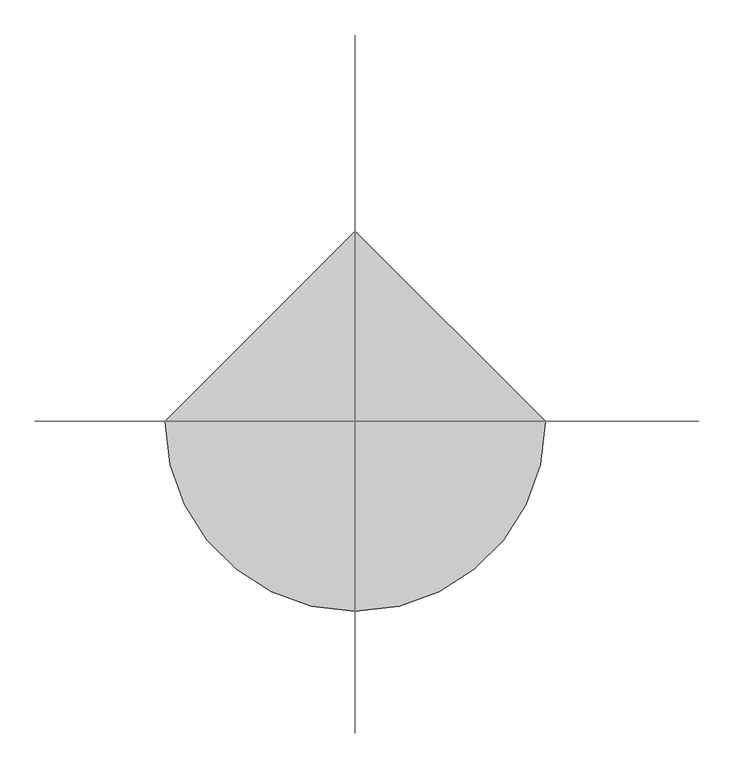
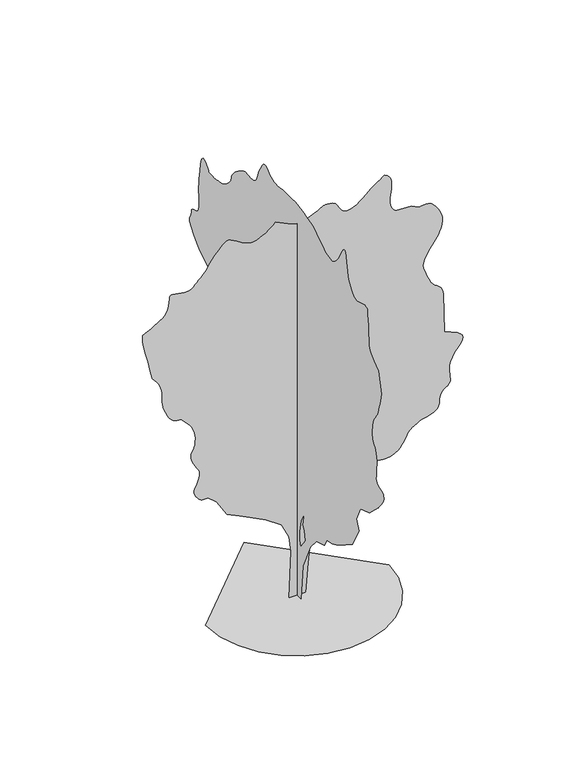
"""IFC4 building model written with IfcOpenShell, lengths in millimetres: proxy geometry, honeylocust 26170 : honeylocust 26170."""

from ifc_helpers import new_model, si_unit, origin, place, context, project, spatial, triangles, source, transform, mapped, element, save


def entourage_cc46a1f1(model_context):
    return source(origin(), model_context, "Body", "Tessellation", [
        triangles([(0.0017564, 138.2462219, 0.0), (0.0017564, -127.0105432, 0.0), (0.0017564, -184.6753374, 668.9082985), (0.0017564, -426.8668951, 1176.3566122), (0.0017564, -611.3926231, 1395.4822632), (0.0017564, -865.1155083, 1476.2135273), (0.0017564, -934.3152088, 1614.6078415), (0.0017564, -1118.8409369, 1660.7391827), (0.0017564, -1168.1321142, 1679.0297813), (0.0017564, -1234.9772346, 1712.4509972), (0.0017564, -1316.4476978, 1758.4833618), (0.0017564, -1409.6173016, 1814.6021748), (0.0017564, -1511.5651485, 1878.2849155), (0.0017564, -1619.3626385, 1947.0122612), (0.0017564, -1730.0862579, 2018.2590752), (0.0017564, -1937.6776566, 2398.8447109), (0.0017564, -1856.9463924, 2583.3806854), (0.0017564, -1983.8091431, 2848.632518), (0.0017564, -2272.1318058, 2952.4168808), (0.0017564, -2537.389016, 3206.1371498), (0.0017564, -2543.9089668, 3214.0110878), (0.0017564, -2561.3334846, 3235.1946785), (0.0017564, -2586.4031754, 3266.0558762), (0.0017564, -2615.9435234, 3302.9873428), (0.0017564, -2646.6774033, 3342.3317436), (0.0017564, -2675.3794304, 3380.4573235), (0.0017564, -2698.8489281, 3413.7311646), (0.0017564, -2714.4444878, 3444.5414932), (0.0017564, -2721.9882133, 3476.5453537), (0.0017564, -2721.8358971, 3508.1684235), (0.0017564, -2714.4444878, 3537.73377), (0.0017564, -2700.1950668, 3563.6926506), (0.0017564, -2679.4940048, 3584.4190018), (0.0017564, -2652.7226738, 3598.2620522), (0.0017564, -2621.3536583, 3608.345739), (0.0017564, -2588.1556847, 3619.6488281), (0.0017564, -2555.5675575, 3633.3648514), (0.0017564, -2526.024884, 3650.7129204), (0.0017564, -2501.9153091, 3672.9124374), (0.0017564, -2485.67444, 3701.157225), (0.0017564, -2479.7233498, 3736.6663948), (0.0017564, -2481.5749809, 3780.2273987), (0.0017564, -2486.0453476, 3831.0780739), (0.0017564, -2491.5266991, 3887.9740196), (0.0017564, -2496.4008202, 3949.6961243), (0.0017564, -2499.0579254, 4015.0755638), (0.0017564, -2497.8818344, 4082.8426483), (0.0017564, -2491.2575294, 4151.8544243), (0.0017564, -2477.5720276, 4213.7541344), (0.0017564, -2458.0368828, 4262.9284584), (0.0017564, -2435.2733013, 4302.24757), (0.0017564, -2411.9053963, 4334.4801956), (0.0017564, -2390.5542286, 4362.4965088), (0.0017564, -2373.8434753, 4389.0902344), (0.0017564, -2364.3947788, 4417.1062569), (0.0017564, -2359.5864967, 4450.1263344), (0.0017564, -2355.5860142, 4489.1913918), (0.0017564, -2353.1983692, 4533.3113731), (0.0017564, -2353.2315067, 4581.4694801), (0.0017564, -2356.4927902, 4632.6250786), (0.0017564, -2363.7901646, 4685.8128204), (0.0017564, -2375.9288132, 4740.016198), (0.0017564, -2392.0679443, 4787.9461212), (0.0017564, -2410.4271435, 4825.3601166), (0.0017564, -2430.3991802, 4855.916391), (0.0017564, -2451.3794403, 4883.2722794), (0.0017564, -2472.7636002, 4911.0089584), (0.0017564, -2493.9471909, 4942.7843445), (0.0017564, -2514.3232727, 4982.2051941), (0.0017564, -2534.0944496, 5031.4045166), (0.0017564, -2553.8659172, 5089.0626251), (0.0017564, -2573.6269203, 5153.8075104), (0.0017564, -2593.4135033, 5224.1654251), (0.0017564, -2613.1747971, 5298.7905212), (0.0017564, -2632.9360909, 5376.2096329), (0.0017564, -2652.7226738, 5455.0763306), (0.0017564, -2548.9127312, 5835.6443802), (0.0017564, -2410.52612, 5939.4537415), (0.0017564, -2376.165136, 5966.8602081), (0.0017564, -2343.2136589, 5995.5625259), (0.0017564, -2313.0867188, 6026.9059616), (0.0017564, -2287.1965839, 6062.1863663), (0.0017564, -2266.9553776, 6102.6995911), (0.0017564, -2253.772752, 6149.7659042), (0.0017564, -2249.0662079, 6204.705574), (0.0017564, -2247.7225399, 6269.3992996), (0.0017564, -2243.9556187, 6343.7709229), (0.0017564, -2238.1721054, 6426.2187973), (0.0017564, -2230.7756092, 6515.1186035), (0.0017564, -2222.1675591, 6608.8704391), (0.0017564, -2212.7518547, 6705.8220795), (0.0017564, -2202.9347214, 6804.4247818), (0.0017564, -2185.5179066, 6814.1270966), (0.0017564, -2167.3950302, 6822.8393555), (0.0017564, -2147.8598854, 6829.5453415), (0.0017564, -2126.2064106, 6833.2026764), (0.0017564, -2101.7285442, 6832.8218857), (0.0017564, -2073.7199341, 6827.4117508), (0.0017564, -2041.4746639, 6815.9560547), (0.0017564, -2006.8748863, 6801.3255524), (0.0017564, -1972.2775795, 6787.914743), (0.0017564, -1937.6776566, 6776.9165771), (0.0017564, -1903.077879, 6769.5501663), (0.0017564, -1868.4805721, 6767.0357849), (0.0017564, -1833.8806492, 6770.5663834), (0.0017564, -1799.2833424, 6781.3616547), (0.0017564, -1765.6919334, 6801.5546082), (0.0017564, -1733.9191635, 6831.4504578), (0.0017564, -1703.6576385, 6869.42314), (0.0017564, -1674.6050514, 6913.8221741), (0.0017564, -1646.4618565, 6963.0982361), (0.0017564, -1618.9257465, 7015.5746841), (0.0017564, -1591.689473, 7069.6766144), (0.0017564, -1522.4922432, 7484.8646439), (0.0017564, -1510.0182953, 7494.262326), (0.0017564, -1496.8382858, 7500.8665741), (0.0017564, -1482.2460079, 7501.8060516), (0.0017564, -1465.5354, 7494.262326), (0.0017564, -1446.0002552, 7475.4413818), (0.0017564, -1422.9345119, 7442.4974625), (0.0017564, -1395.6321087, 7392.5865555), (0.0017564, -1366.480545, 7335.9952423), (0.0017564, -1337.5296959, 7284.4588531), (0.0017564, -1307.5703327, 7237.3669601), (0.0017564, -1275.393663, 7194.085881), (0.0017564, -1239.7855167, 7154.0296051), (0.0017564, -1199.5366653, 7116.6156097), (0.0017564, -1153.4407871, 7081.2078873), (0.0017564, -1100.9873028, 7057.7133911), (0.0017564, -1043.0880753, 7054.1827927), (0.0017564, -980.6472645, 7067.2889694), (0.0017564, -914.5768787, 7093.7047989), (0.0017564, -845.7836214, 7130.1287384), (0.0017564, -775.1741959, 7173.2069229), (0.0017564, -703.6555235, 7219.6128113), (0.0017564, -659.2741482, 7251.5405136), (0.0017564, -615.4946983, 7282.3758408), (0.0017564, -572.9269114, 7311.0014191), (0.0017564, -532.1751838, 7336.2748764), (0.0017564, -493.8440932, 7357.1282547), (0.0017564, -458.5406522, 7372.4186005), (0.0017564, -426.8668951, 7381.0547012), (0.0017564, -379.7931333, 7391.6464966), (0.0017564, -304.4771091, 7410.7220764), (0.0017564, -210.8004869, 7434.013678), (0.0017564, -108.6519436, 7457.3308594), (0.0017564, -7.915369, 7476.3808594), (0.0017564, 81.5235032, 7486.9726547), (0.0017564, 149.779584, 7484.8646439), (0.0017564, 204.0816928, 7478.1336594), (0.0017564, 257.9799291, 7476.2541229), (0.0017564, 311.0709472, 7476.9907059), (0.0017564, 362.9529548, 7478.1336594), (0.0017564, 413.2194723, 7477.4732346), (0.0017564, 461.4692888, 7472.7485229), (0.0017564, 507.2984682, 7461.8015167), (0.0017564, 555.4821914, 7451.6666702), (0.0017564, 608.9110522, 7450.0156082), (0.0017564, 664.3541433, 7455.4513229), (0.0017564, 718.5906584, 7466.5000671), (0.0017564, 768.3873281, 7481.7909943), (0.0017564, 810.5182594, 7499.9265152), (0.0017564, 841.7526175, 7519.4590439), (0.0017564, 869.6950979, 7543.2081757), (0.0017564, 902.8827524, 7570.9704346), (0.0017564, 939.4967966, 7596.9293152), (0.0017564, 977.728838, 7615.2171524), (0.0017564, 1015.7551506, 7619.9924423), (0.0017564, 1051.7671967, 7605.3875198), (0.0017564, 1083.943939, 7565.5858795), (0.0017564, 1111.584185, 7516.9952408), (0.0017564, 1135.5896965, 7477.701709), (0.0017564, 1156.5725727, 7444.2496811), (0.0017564, 1175.132341, 7413.2114594), (0.0017564, 1191.8760138, 7381.1564392), (0.0017564, 1207.410676, 7344.6819214), (0.0017564, 1222.3407967, 7300.3334656), (0.0017564, 1236.6967518, 7254.9693741), (0.0017564, 1251.0554684, 7217.07285), (0.0017564, 1266.8236919, 7185.6526749), (0.0017564, 1285.4164524, 7159.6432159), (0.0017564, 1308.248489, 7138.103833), (0.0017564, 1336.7269833, 7119.9683121), (0.0017564, 1372.2666744, 7104.2710144), (0.0017564, 1413.6914715, 7095.1529663), (0.0017564, 1457.9408054, 7094.9239105), (0.0017564, 1503.6022625, 7099.7247803), (0.0017564, 1549.2612488, 7105.7447617), (0.0017564, 1593.5105827, 7109.1480423), (0.0017564, 1634.9353798, 7106.0999725), (0.0017564, 1672.1235168, 7092.7397415), (0.0017564, 1714.3205051, 7068.3051865), (0.0017564, 1768.2192501, 7035.5897415), (0.0017564, 1828.5747231, 6996.1944717), (0.0017564, 1890.1391338, 6951.7954376), (0.0017564, 1947.6700699, 6903.9419632), (0.0017564, 1995.9198864, 6854.2845291), (0.0017564, 2029.6434093, 6804.4247818), (0.0017564, 2047.5985634, 6762.5657089), (0.0017564, 2056.0720287, 6732.1873306), (0.0017564, 2061.1140175, 6707.879512), (0.0017564, 2068.7821541, 6684.1809586), (0.0017564, 2085.1219997, 6655.6315384), (0.0017564, 2116.1913242, 6616.7949554), (0.0017564, 2168.0377235, 6562.2360764), (0.0017564, 2230.1762272, 6507.9306702), (0.0017564, 2288.0754547, 6470.9736237), (0.0017564, 2341.7380222, 6447.5297058), (0.0017564, 2391.1637844, 6433.7881027), (0.0017564, 2436.3553574, 6425.8885849), (0.0017564, 2477.3077995, 6419.9959213), (0.0017564, 2514.0259071, 6412.2998795), (0.0017564, 2553.510125, 6405.0352066), (0.0017564, 2599.6366699, 6402.2161926), (0.0017564, 2647.7694878, 6402.6225632), (0.0017564, 2693.3117661, 6405.0352066), (0.0017564, 2731.5640823, 6408.2611725), (0.0017564, 2757.9293335, 6411.0807678), (0.0017564, 2767.7589661, 6412.2998795), (0.0017564, 2779.3922676, 6430.4609802), (0.0017564, 2809.9738312, 6472.8281616), (0.0017564, 2853.0775955, 6521.2403229), (0.0017564, 2902.2519196, 6557.5625244), (0.0017564, 2950.9945839, 6563.6075043), (0.0017564, 2992.9045258, 6521.2403229), (0.0017564, 3021.4792351, 6412.2998795), (0.0017564, 3039.1830963, 6281.2613663), (0.0017564, 3053.0770157, 6180.2965988), (0.0017564, 3063.5417839, 6102.7251709), (0.0017564, 3070.9584824, 6041.8916748), (0.0017564, 3075.7846413, 5991.1680267), (0.0017564, 3078.3751808, 5943.8482407), (0.0017564, 3079.1373436, 5893.3274872), (0.0017564, 3077.918232, 5838.9459229), (0.0017564, 3075.0986366, 5784.5899384), (0.0017564, 3071.8729614, 5730.2089554), (0.0017564, 3069.4600273, 5675.8273911), (0.0017564, 3069.0536568, 5621.4714066), (0.0017564, 3071.8729614, 5567.0904236), (0.0017564, 3079.1373436, 5512.7344391), (0.0017564, 3099.1779808, 5469.782991), (0.0017564, 3134.966494, 5444.6112717), (0.0017564, 3179.5942932, 5429.5238205), (0.0017564, 3226.2792343, 5416.8495941), (0.0017564, 3268.113018, 5398.9169678), (0.0017564, 3298.2376328, 5368.0816406), (0.0017564, 3309.7944855, 5316.6719879), (0.0017564, 3318.6843498, 5264.1193817), (0.0017564, 3338.4456436, 5228.1023941), (0.0017564, 3358.8164932, 5198.3588608), (0.0017564, 3369.5097359, 5164.551622), (0.0017564, 3360.2387901, 5116.4440933), (0.0017564, 3320.6912041, 5043.7235321), (0.0017564, 3240.6051041, 4936.0789398), (0.0017564, 3137.9128258, 4824.090136), (0.0017564, 3039.0560692, 4740.5243065), (0.0017564, 2946.4477684, 4678.5737274), (0.0017564, 2862.5264374, 4631.3298088), (0.0017564, 2789.7047195, 4591.9598282), (0.0017564, 2730.395549, 4553.5804848), (0.0017564, 2687.0124413, 4509.3590561), (0.0017564, 2658.1580978, 4464.7821259), (0.0017564, 2638.3970947, 4426.6568367), (0.0017564, 2624.0715157, 4390.1317406), (0.0017564, 2611.574604, 4350.4059677), (0.0017564, 2597.249025, 4302.5777824), (0.0017564, 2577.462442, 4241.8466057), (0.0017564, 2548.6333878, 4163.3859879), (0.0017564, 2517.7242279, 4078.1182274), (0.0017564, 2493.4823936, 3999.5052933), (0.0017564, 2474.7855698, 3926.4298119), (0.0017564, 2460.5312073, 3857.7988266), (0.0017564, 2449.6039673, 3792.521125), (0.0017564, 2440.8943245, 3729.4275925), (0.0017564, 2433.294643, 3667.4770134), (0.0017564, 2455.3521629, 3642.6102173), (0.0017564, 2476.2994308, 3616.9562599), (0.0017564, 2495.0267761, 3589.7021095), (0.0017564, 2510.4267082, 3560.0097359), (0.0017564, 2521.3894112, 3527.0913963), (0.0017564, 2526.8021622, 3490.1343498), (0.0017564, 2525.5600868, 3448.3514351), (0.0017564, 2526.3652702, 3406.9748909), (0.0017564, 2533.4264671, 3370.2718987), (0.0017564, 2538.8723557, 3335.7786552), (0.0017564, 2534.8385902, 3301.0569374), (0.0017564, 2513.4544304, 3263.7443893), (0.0017564, 2466.850589, 3221.3772079), (0.0017564, 2387.1633018, 3171.5424591), (0.0017564, 2299.4063038, 3131.0039452), (0.0017564, 2230.2092194, 3111.2173622), (0.0017564, 2174.1235439, 3101.9464165), (0.0017564, 2125.7061504, 3092.878656), (0.0017564, 2079.5060635, 3073.7016289), (0.0017564, 2030.0803013, 3034.1540428), (0.0017564, 1971.9778885, 2963.9484444), (0.0017564, 1918.922406, 2886.046804), (0.0017564, 1885.02869, 2826.5091591), (0.0017564, 1865.4579369, 2779.671611), (0.0017564, 1855.3716339, 2739.8952599), (0.0017564, 1849.9258907, 2701.5159164), (0.0017564, 1844.2769623, 2658.9202606), (0.0017564, 1833.5835743, 2606.4438126), (0.0017564, 1823.3625412, 2556.2026932), (0.0017564, 1818.1834969, 2520.8993248), (0.0017564, 1811.7953693, 2495.6822594), (0.0017564, 1797.9422905, 2475.7102226), (0.0017564, 1770.3705723, 2456.1393242), (0.0017564, 1722.8269627, 2432.1339581), (0.0017564, 1649.0577736, 2398.8447109), (0.0017564, 1567.2851486, 2366.9372108), (0.0017564, 1497.6180347, 2346.9297112), (0.0017564, 1436.6226299, 2333.7851646), (0.0017564, 1380.8747246, 2322.4516994), (0.0017564, 1326.9429874, 2307.8950298), (0.0017564, 1271.3957966, 2285.0629932), (0.0017564, 1210.806617, 2248.9188332), (0.0017564, 1144.870816, 2202.0812851), (0.0017564, 1075.9099091, 2151.0044609), (0.0017564, 1004.4242289, 2096.4021252), (0.0017564, 930.9242821, 2038.9727818), (0.0017564, 855.9105469, 1979.4251083), (0.0017564, 779.8858995, 1918.4651665), (0.0017564, 703.3583033, 1856.7991631), (0.0017564, 276.64129, 1533.8765774), (0.0017564, 149.779584, 1314.7509991), (0.0017564, 115.1805058, 1141.7593054), (0.0017564, 103.6476433, 876.5023132), (0.0020752, -103.9448272, 980.2967772), (0.0020752, -80.8791112, 1107.1595278), (0.0020752, -80.8791112, 1268.6195126), (0.0020752, -127.0105432, 1499.2792706), (0.0020752, -230.8067694, 1706.8706692), (0.0020752, -184.6753374, 1453.147784), (0.0020752, -230.8067694, 1372.4165199), (0.0020752, -265.4043305, 1199.4223555), (154.7882082, 0.0004434, 0.0162828), (-145.0671264, 0.0004434, 0.0162828), (-110.4685569, 0.0003925, 876.5175739), (-145.0671264, 0.000378, 1164.8403093), (-283.4611681, 0.0003635, 1441.6288651), (-560.2523217, 0.0003489, 1637.6887001), (-963.9036644, 0.0003344, 1845.2827148), (-1263.7605068, 0.0003271, 1983.677029), (-1459.8203419, 0.0003126, 2295.065435), (-1609.7462196, 0.000298, 2421.9281857), (-1636.8810459, 0.0003053, 2419.6396626), (-1663.7135651, 0.0003053, 2418.4637169), (-1689.9389992, 0.0003053, 2419.5050777), (-1715.2578026, 0.000298, 2423.8764679), (-1739.3649067, 0.000298, 2432.6877033), (-1761.9606205, 0.000298, 2447.0436584), (-1782.7404568, 0.000298, 2468.0595268), (-1802.9155334, 0.000298, 2493.4774521), (-1822.6843849, 0.000298, 2520.3098259), (-1840.2357845, 0.0002908, 2548.5572296), (-1853.7537094, 0.0002908, 2578.199025), (-1861.4193752, 0.0002908, 2609.2886971), (-1861.4193752, 0.0002908, 2641.7497971), (-1851.9375412, 0.0002835, 2675.6587738), (-1833.5784874, 0.0002835, 2714.1904335), (-1810.985099, 0.0002835, 2759.3769196), (-1788.3893852, 0.0002762, 2809.4148537), (-1770.0301861, 0.0002762, 2862.4755684), (-1760.1445976, 0.000269, 2916.7298149), (-1762.9689892, 0.000269, 2970.4000854), (-1782.7404568, 0.000269, 3021.631842), (-1812.8012672, 0.0002617, 3069.7646599), (-1842.4557072, 0.0002617, 3115.6624397), (-1869.8928406, 0.0002544, 3159.9347374), (-1893.2963539, 0.0002544, 3203.2161072), (-1910.8477535, 0.0002544, 3246.0658173), (-1920.7308712, 0.0002471, 3289.1442924), (-1921.134771, 0.0002471, 3333.0355087), (-1913.6366821, 0.0002471, 3370.6526894), (-1902.1049732, 0.0002399, 3398.1864738), (-1888.1503017, 0.0002399, 3421.0972847), (-1873.3903015, 0.0002399, 3444.7952568), (-1859.43563, 0.0002399, 3474.7419754), (-1847.9014503, 0.0002399, 3516.397863), (-1840.4059776, 0.0002326, 3575.2242142), (-1839.1614315, 0.0002253, 3640.3751793), (-1844.5740372, 0.0002253, 3698.2870514), (-1855.534124, 0.0002253, 3750.1283638), (-1870.9342014, 0.0002181, 3797.143808), (-1889.6641628, 0.0002181, 3840.5016266), (-1910.6114307, 0.0002181, 3881.4718002), (-1932.6688053, 0.0002108, 3921.1972824), (-2094.1288628, 0.0002035, 4094.1966064), (-2131.1822697, 0.0002035, 4094.6791351), (-2168.1342293, 0.0002035, 4097.9556793), (-2204.8854744, 0.0002035, 4106.8964127), (-2241.3344124, 0.0002035, 4124.3209305), (-2277.3769798, 0.0001963, 4153.0482468), (-2312.9191418, 0.0001963, 4195.8726677), (-2347.8542187, 0.000189, 4255.6640762), (-2378.9895275, 0.000189, 4321.6024933), (-2403.4675392, 0.0001817, 4382.0799065), (-2421.6893921, 0.0001817, 4438.7470871), (-2434.0643635, 0.0001817, 4493.1792297), (-2440.9908302, 0.0001745, 4547.0018166), (-2442.8729828, 0.0001745, 4601.8403297), (-2440.1170464, 0.0001672, 4659.3205421), (-2439.9138611, 0.0001672, 4717.8166809), (-2448.3874718, 0.0001599, 4774.3062561), (-2464.3234177, 0.0001599, 4828.1797119), (-2486.5177025, 0.0001527, 4878.801622), (-2513.751796, 0.0001527, 4925.6138809), (-2544.8234459, 0.0001527, 4967.9810623), (-2578.5039482, 0.0001454, 5005.2933197), (-2606.1136002, 0.0001454, 5036.2053864), (-2622.8268242, 0.0001454, 5064.6786484), (-2633.2915924, 0.0001454, 5098.2068344), (-2642.1308784, 0.0001381, 5144.2313507), (-2653.9926544, 0.0001381, 5210.2459259), (-2673.5251831, 0.0001308, 5303.6669678), (-2705.3767273, 0.0001236, 5432.0132034), (-2739.5397583, 0.0001163, 5564.8295151), (-2764.0251823, 0.000109, 5669.807991), (-2780.4334831, 0.0001018, 5751.5704422), (-2790.3651443, 0.0001018, 5814.7910019), (-2795.4959358, 9.45e-05, 5864.0920624), (-2797.3754723, 9.45e-05, 5904.0971786), (-2797.6295265, 9.45e-05, 5939.4537415), (-2780.0526924, 9.45e-05, 5947.0736252), (-2760.7486382, 9.45e-05, 5955.7608856), (-2738.0157234, 8.72e-05, 5966.7078918), (-2710.1520172, 8.72e-05, 5980.9576035), (-2675.4047195, 8.72e-05, 5999.6518112), (-2632.0977699, 8.72e-05, 6023.8834717), (-2578.5039482, 8.72e-05, 6054.794957), (-2522.6948547, 8e-05, 6086.4941849), (-2473.739122, 8e-05, 6114.9674469), (-2431.4405411, 8e-05, 6144.0761353), (-2395.5985428, 8e-05, 6177.5787415), (-2366.0102325, 7.27e-05, 6219.387236), (-2342.4746052, 7.27e-05, 6273.2856903), (-2324.7886208, 6.54e-05, 6343.110498), (-2314.1282249, 6.54e-05, 6412.6556717), (-2308.7154739, 5.82e-05, 6464.4205353), (-2303.9071918, 5.82e-05, 6500.4631027), (-2295.0629642, 5.82e-05, 6522.7896469), (-2277.5471729, 5.82e-05, 6533.4320206), (-2246.7141712, 5.82e-05, 6534.3720795), (-2197.9258701, 5.82e-05, 6527.641095), (-2140.092627, 5.82e-05, 6517.4300903), (-2085.4878204, 5.82e-05, 6508.0068283), (-2034.5150597, 5.82e-05, 6501.6060562), (-1987.575919, 5.82e-05, 6500.4631027), (-1945.0767689, 5.82e-05, 6506.7877167), (-1907.4187477, 5.82e-05, 6522.7896469), (-1875.0032845, 5.82e-05, 6550.7042221), (-1844.541045, 5.09e-05, 6583.0894547), (-1812.0595974, 5.09e-05, 6613.4422531), (-1776.9567982, 5.09e-05, 6645.4205338), (-1738.6257076, 5.09e-05, 6682.6572144), (-1696.4617115, 4.36e-05, 6728.7578888), (-1649.8604862, 4.36e-05, 6787.3560562), (-1598.2146561, 3.63e-05, 6862.1078888), (-1546.1980637, 2.91e-05, 6938.7142593), (-1498.4181313, 2.91e-05, 7002.036557), (-1454.1714134, 2.91e-05, 7054.2589508), (-1412.7466164, 2.18e-05, 7097.5911896), (-1373.4401493, 2.18e-05, 7134.268602), (-1335.5459507, 2.18e-05, 7166.5265167), (-1298.3578136, 1.45e-05, 7196.5496841), (-1288.0707962, 1.45e-05, 7208.5129074), (-1275.3606709, 1.45e-05, 7218.1646439), (-1257.8092712, 1.45e-05, 7223.193988), (-1232.9934895, 1.45e-05, 7221.2382935), (-1198.4952318, 1.45e-05, 7210.0116531), (-1151.8939339, 1.45e-05, 7187.1770004), (-1090.7663424, 2.18e-05, 7150.4228485), (-1026.7456861, 2.18e-05, 7109.5544128), (-971.2010387, 2.18e-05, 7076.382019), (-921.3027763, 2.91e-05, 7051.4649353), (-874.2290508, 2.91e-05, 7035.4374252), (-827.1577961, 2.91e-05, 7028.858757), (-777.2595337, 2.91e-05, 7032.3893555), (-721.7123428, 2.91e-05, 7046.6134872), (-664.755427, 2.18e-05, 7068.7365555), (-612.0327003, 2.18e-05, 7095.1018066), (-562.8405722, 2.18e-05, 7124.9976563), (-516.4729082, 2.18e-05, 7157.7131012), (-472.226154, 1.45e-05, 7192.5615555), (-429.3891249, 1.45e-05, 7228.8075989), (-387.2581573, 1.45e-05, 7265.7390656), (-168.1328515, 2.18e-05, 7161.9547028), (-133.3996518, 2.18e-05, 7144.8603973), (-97.8597517, 2.18e-05, 7129.1125214), (-60.7056832, 2.18e-05, 7115.9551849), (-21.1306711, 2.18e-05, 7106.7348175), (21.6722237, 2.18e-05, 7102.77285), (68.5100806, 2.18e-05, 7105.3633896), (120.1896296, 2.18e-05, 7115.8284485), (179.9390167, 2.18e-05, 7135.6656097), (246.5473965, 2.18e-05, 7162.9709198), (314.1646537, 1.45e-05, 7193.9079849), (376.9406911, 1.45e-05, 7224.6165756), (429.0233405, 1.45e-05, 7251.3120392), (464.5629953, 1.45e-05, 7270.1585632), (477.7100126, 1.45e-05, 7277.2703384), (487.5271096, 1.45e-05, 7279.4550888), (513.8897447, 1.45e-05, 7283.4682159), (552.1522711, 1.45e-05, 7285.4494904), (597.6791797, 1.45e-05, 7281.5886795), (645.8273672, 1.45e-05, 7268.0249725), (691.9587811, 1.45e-05, 7240.9737167), (731.4328978, 1.45e-05, 7196.5496841), (761.0238968, 2.18e-05, 7148.2642593), (783.1472557, 2.18e-05, 7111.0787384), (801.640967, 2.18e-05, 7083.3670578), (820.3353928, 2.18e-05, 7063.5298965), (843.065764, 2.91e-05, 7049.9406097), (873.6625883, 2.91e-05, 7040.9998764), (915.9611692, 2.91e-05, 7035.081633), (967.9092339, 2.91e-05, 7039.3999741), (1023.6901314, 2.18e-05, 7059.6435059), (1081.4903097, 2.18e-05, 7091.9775787), (1139.4911299, 2.18e-05, 7132.5925415), (1195.8764963, 1.45e-05, 7177.6520004), (1248.8354004, 1.45e-05, 7223.3207245), (1296.5467323, 1.45e-05, 7265.7390656), (1340.3591743, 7.3e-06, 7303.2803787), (1382.9600624, 7.3e-06, 7337.1637756), (1424.5524364, 7.3e-06, 7368.0246826), (1465.3373016, 7.3e-06, 7396.4723648), (1505.5174072, 0.0, 7423.1172501), (1545.2937584, 0.0, 7448.5168625), (1584.8695404, 0.0, 7473.3327896), (1611.8696365, 0.0, 7460.5568253), (1637.7599167, 0.0, 7445.2658981), (1661.4301289, 0.0, 7424.9206284), (1681.7729279, 7.3e-06, 7397.0060532), (1697.6758816, 7.3e-06, 7359.0327896), (1708.0339703, 7.3e-06, 7308.4108795), (1711.732291, 1.45e-05, 7242.6759384), (1708.6384392, 2.18e-05, 7173.2069229), (1701.1073582, 2.18e-05, 7112.0182159), (1691.7602543, 2.18e-05, 7057.4843353), (1683.2181885, 2.91e-05, 7007.9797989), (1678.1077446, 2.91e-05, 6961.9297028), (1679.0501289, 3.63e-05, 6917.6829849), (1688.6665478, 3.63e-05, 6873.639743), (1703.4950031, 3.63e-05, 6833.8631012), (1718.3209877, 4.36e-05, 6802.5452454), (1733.1494431, 4.36e-05, 6778.3135849), (1747.9780437, 4.36e-05, 6759.7205338), (1762.8064991, 4.36e-05, 6745.3440857), (1777.6324837, 4.36e-05, 6733.8128128), (1792.460939, 4.36e-05, 6723.7035461), (2069.2520382, 4.36e-05, 6712.1716919), (2207.6463524, 5.09e-05, 6642.9823105), (2217.499094, 5.09e-05, 6645.8524841), (2244.0954357, 5.09e-05, 6651.9742035), (2282.9953869, 5.09e-05, 6657.485495), (2329.7669506, 5.09e-05, 6658.5778702), (2379.9675201, 5.09e-05, 6651.3899368), (2429.1595757, 5.09e-05, 6632.0858826), (2472.9034172, 5.09e-05, 6596.8304764), (2512.6797684, 5.82e-05, 6549.0025818), (2551.0463219, 5.82e-05, 6495.1035461), (2585.1840637, 6.54e-05, 6436.1501678), (2612.2350288, 6.54e-05, 6373.1836624), (2629.4307816, 7.27e-05, 6307.1690872), (2633.9011482, 7.27e-05, 6239.1482391), (2622.8268242, 8e-05, 6170.111174), (2602.049604, 8e-05, 6105.620343), (2579.4690056, 8.72e-05, 6049.6132965), (2555.3390831, 8.72e-05, 6000.6680283), (2530.0304535, 8.72e-05, 5957.360788), (2503.8024033, 9.45e-05, 5918.2701508), (2476.9726456, 9.45e-05, 5882.0246887), (2449.837674, 9.45e-05, 5847.2012329), (2408.2121624, 0.0001018, 5785.5299973), (2368.9058407, 0.0001018, 5724.5703461), (2334.2399334, 0.000109, 5665.0327011), (2306.5336304, 0.000109, 5607.603067), (2288.1084469, 0.0001163, 5552.9930283), (2281.2834274, 0.0001163, 5501.9141693), (2288.3777618, 0.0001236, 5455.0763306), (2303.2722015, 0.0001236, 5411.8202499), (2318.5706863, 0.0001236, 5370.1390732), (2334.6768253, 0.0001308, 5328.8892654), (2351.9919022, 0.0001308, 5286.8267166), (2370.922578, 0.0001308, 5242.7578949), (2391.869846, 0.0001381, 5195.4375275), (2415.2378963, 0.0001381, 5143.6982437), (2445.5678764, 0.0001454, 5097.4190918), (2484.1684273, 0.0001454, 5063.0531662), (2526.5989769, 0.0001454, 5034.1479538), (2568.4199707, 0.0001454, 5004.2265244), (2605.2247009, 0.0001527, 4966.8381088), (2632.5041405, 0.0001527, 4915.5301941), (2645.8899513, 0.0001599, 4843.8258499), (2668.9530785, 0.0002035, 4105.72817), (2899.6102203, 0.0002108, 4001.9438072), (2935.957711, 0.0002108, 3979.3123398), (2967.9871513, 0.0002108, 3954.3696762), (2991.3043327, 0.0002108, 3924.7787498), (3001.6420738, 0.0002108, 3888.2280739), (2994.6061661, 0.0002181, 3842.381163), (2965.9041389, 0.0002181, 3784.9518196), (2911.1417839, 0.0002253, 3713.6032677), (2850.7916885, 0.0002326, 3637.2509514), (2806.7987343, 0.0002326, 3565.9279793), (2777.1063606, 0.0002399, 3499.049794), (2759.707132, 0.0002399, 3436.0068398), (2752.6206459, 0.0002471, 3376.1901421), (2753.7891792, 0.0002471, 3319.0145622), (2761.2311668, 0.0002544, 3263.8205475), (2769.4861862, 0.0002544, 3214.1381149), (2773.7280785, 0.0002544, 3172.7107018), (2772.7374413, 0.0002617, 3137.9384056), (2765.2698738, 0.0002617, 3108.2201614), (2750.1315536, 0.0002617, 3081.9313591), (2726.1283676, 0.0002617, 3057.4456444), (2692.0162056, 0.0002617, 3033.1634056), (2656.5834846, 0.000269, 3007.7126335), (2628.8212257, 0.000269, 2980.6616684), (2607.8916893, 0.000269, 2951.756456), (2593.0327126, 0.000269, 2920.8699692), (2583.4315544, 0.0002762, 2887.7484444), (2578.249894, 0.0002762, 2852.2139854), (2576.7002792, 0.0002762, 2814.0378273), (2574.4905304, 0.0002835, 2776.5473831), (2567.4293335, 0.0002835, 2742.8924606), (2554.9071327, 0.0002835, 2712.6663986), (2536.3501259, 0.0002835, 2685.4631172), (2511.1330605, 0.0002908, 2660.9012444), (2478.6539383, 0.0002908, 2638.5238312), (2438.3036396, 0.0002908, 2617.9753761), (2396.3758209, 0.0002908, 2601.9734459), (2358.4816223, 0.0002908, 2591.6357048), (2323.0080608, 0.0002908, 2584.0916885), (2288.3421535, 0.0002908, 2576.5735428), (2252.8710629, 0.0002908, 2566.2102219), (2214.9768642, 0.0002908, 2550.2082916), (2173.0465748, 0.000298, 2525.7225769), (2134.3801849, 0.000298, 2501.648465), (2105.1956291, 0.000298, 2485.6439186), (2082.2644707, 0.000298, 2473.0685234), (2062.3585636, 0.000298, 2459.2838997), (2042.2519421, 0.000298, 2439.6473076), (2018.7163147, 0.0003053, 2409.5203674), (1988.5207741, 0.0003053, 2364.2626648), (1957.3856106, 0.0003053, 2310.7346821), (1930.083062, 0.0003126, 2259.4242966), (1901.9730045, 0.0003126, 2211.1414879), (1868.4170586, 0.0003198, 2166.6889687), (1824.7748096, 0.0003198, 2126.8796253), (1766.4030819, 0.0003198, 2092.5158798), (1688.6665478, 0.0003198, 2064.4058224), (1611.2981598, 0.0003271, 2049.7144226), (1552.6928707, 0.0003271, 2049.9481293), (1506.1906219, 0.0003198, 2057.4462181), (1465.1365871, 0.0003198, 2064.5404072), (1422.8709984, 0.0003198, 2063.5676468), (1372.7390293, 0.0003271, 2046.8544228), (1308.0784412, 0.0003271, 2006.7427723), (1236.0922829, 0.0003271, 1957.583709), (1168.5411009, 0.0003344, 1917.1011509), (1105.630406, 0.0003344, 1882.6715664), (1047.5635288, 0.0003344, 1851.6708424), (994.5385677, 0.0003344, 1821.4753017), (946.7611788, 0.0003416, 1789.4663544), (904.4270622, 0.0003416, 1753.0174164), (863.5407497, 0.0003416, 1713.1393272), (820.2337275, 0.0003489, 1672.6569145), (774.9100405, 0.0003489, 1631.6714802), (727.9708998, 0.0003489, 1590.2796753), (679.8201324, 0.0003562, 1548.5857086), (630.8642544, 0.0003562, 1506.6908821), (581.50702, 0.0003562, 1464.6946083), (339.3157348, 0.000378, 1176.3718729), (235.5192361, 0.0003925, 899.5832445), (200.9196402, 0.0004143, 542.0633883), (-1658.5903313, 0.0, 0.0172132), (-1614.7424263, -380.0394845, 0.0172132), (-1489.866037, -729.0453255, 0.0172132), (-1293.9560474, -1037.0174429, 0.0172132), (-1037.0174429, -1293.9560474, 0.0172132), (-729.0453255, -1489.866037, 0.0172132), (-380.0394845, -1614.7424263, 0.0172132), (7.25e-05, -1658.5903313, 0.0172132), (380.0394845, -1614.7424263, 0.0172132), (729.0453255, -1489.866037, 0.0172132), (1037.0174429, -1293.9560474, 0.0172132), (1293.9560474, -1037.0174429, 0.0172132), (1489.866037, -729.0453255, 0.0172132), (1614.7424263, -380.0394845, 0.0172132), (1658.5903313, 0.0001454, 0.0172132), (-0.0002175, 1658.5903313, 0.0172132)], [[328, 1, 329], [327, 328, 329], [327, 329, 330], [329, 1, 2], [329, 2, 3], [329, 3, 4], [336, 329, 4], [327, 330, 331], [326, 327, 331], [326, 331, 332], [325, 326, 332], [335, 336, 4], [335, 4, 5], [325, 332, 333], [334, 335, 5], [333, 334, 5], [333, 5, 6], [333, 6, 7], [324, 325, 333], [91, 92, 93], [223, 224, 225], [222, 223, 225], [222, 225, 226], [221, 222, 226], [220, 221, 226], [220, 226, 227], [219, 220, 227], [219, 227, 228], [15, 16, 17], [91, 93, 94], [91, 94, 95], [91, 95, 96], [91, 96, 97], [91, 97, 98], [91, 98, 99], [91, 99, 100], [90, 91, 100], [90, 100, 101], [90, 101, 102], [89, 90, 102], [89, 102, 103], [88, 89, 103], [88, 103, 104], [218, 219, 228], [14, 15, 17], [218, 228, 229], [217, 218, 229], [216, 217, 229], [216, 229, 230], [215, 216, 230], [215, 230, 231], [214, 215, 231], [214, 231, 232], [214, 232, 233], [214, 233, 234], [213, 214, 234], [213, 234, 235], [113, 114, 115], [113, 115, 116], [113, 116, 117], [113, 117, 118], [113, 118, 119], [113, 119, 120], [113, 120, 121], [113, 121, 122], [113, 122, 123], [113, 123, 124], [113, 124, 125], [113, 125, 126], [113, 126, 127], [112, 113, 127], [112, 127, 128], [111, 112, 128], [110, 111, 128], [213, 235, 236], [87, 88, 104], [87, 104, 105], [212, 213, 236], [110, 128, 129], [109, 110, 129], [212, 236, 237], [211, 212, 237], [210, 211, 237], [86, 87, 105], [210, 237, 238], [209, 210, 238], [85, 86, 105], [76, 77, 78], [75, 76, 78], [13, 14, 17], [209, 238, 239], [85, 105, 106], [208, 209, 239], [74, 75, 78], [108, 109, 129], [74, 78, 79], [73, 74, 79], [84, 85, 106], [73, 79, 80], [72, 73, 80], [71, 72, 80], [208, 239, 240], [70, 71, 80], [69, 70, 80], [68, 69, 80], [67, 68, 80], [66, 67, 80], [65, 66, 80], [65, 80, 81], [64, 65, 81], [12, 13, 17], [245, 246, 247], [244, 245, 247], [243, 244, 247], [243, 247, 248], [64, 81, 82], [63, 64, 82], [242, 243, 248], [323, 324, 333], [167, 168, 169], [167, 169, 170], [166, 167, 170], [166, 170, 171], [165, 166, 171], [164, 165, 171], [164, 171, 172], [163, 164, 172], [163, 172, 173], [163, 173, 174], [162, 163, 174], [162, 174, 175], [162, 175, 176], [162, 176, 177], [161, 162, 177], [161, 177, 178], [161, 178, 179], [160, 161, 179], [160, 179, 180], [159, 160, 180], [159, 180, 181], [158, 159, 181], [11, 12, 17], [250, 251, 252], [249, 250, 252], [249, 252, 253], [248, 249, 253], [242, 248, 253], [242, 253, 254], [242, 254, 255], [241, 242, 255], [241, 255, 256], [241, 256, 257], [241, 257, 258], [241, 258, 259], [240, 241, 259], [208, 240, 259], [208, 259, 260], [208, 260, 261], [207, 208, 261], [206, 207, 261], [206, 261, 262], [206, 262, 263], [205, 206, 263], [205, 263, 264], [204, 205, 264], [204, 264, 265], [204, 265, 266], [204, 266, 267], [204, 267, 268], [204, 268, 269], [203, 204, 269], [10, 11, 17], [9, 10, 17], [8, 9, 17], [7, 8, 17], [333, 7, 17], [323, 333, 17], [322, 323, 17], [322, 17, 18], [321, 322, 18], [320, 321, 18], [319, 320, 18], [318, 319, 18], [317, 318, 18], [316, 317, 18], [315, 316, 18], [203, 269, 270], [314, 315, 18], [18, 19, 20], [314, 18, 20], [314, 20, 21], [314, 21, 22], [314, 22, 23], [314, 23, 24], [314, 24, 25], [314, 25, 26], [314, 26, 27], [314, 27, 28], [314, 28, 29], [314, 29, 30], [314, 30, 31], [314, 31, 32], [314, 32, 33], [314, 33, 34], [314, 34, 35], [314, 35, 36], [314, 36, 37], [314, 37, 38], [314, 38, 39], [314, 39, 40], [314, 40, 41], [314, 41, 42], [314, 42, 43], [314, 43, 44], [314, 44, 45], [314, 45, 46], [314, 46, 47], [314, 47, 48], [314, 48, 49], [314, 49, 50], [314, 50, 51], [314, 51, 52], [314, 52, 53], [314, 53, 54], [314, 54, 55], [314, 55, 56], [314, 56, 57], [314, 57, 58], [314, 58, 59], [314, 59, 60], [314, 60, 61], [314, 61, 62], [313, 314, 62], [312, 313, 62], [311, 312, 62], [310, 311, 62], [309, 310, 62], [308, 309, 62], [307, 308, 62], [306, 307, 62], [305, 306, 62], [304, 305, 62], [303, 304, 62], [302, 303, 62], [301, 302, 62], [300, 301, 62], [299, 300, 62], [298, 299, 62], [297, 298, 62], [296, 297, 62], [295, 296, 62], [294, 295, 62], [294, 62, 63], [294, 63, 82], [294, 82, 83], [294, 83, 84], [294, 84, 106], [294, 106, 107], [294, 107, 108], [294, 108, 129], [294, 129, 130], [294, 130, 131], [294, 131, 132], [294, 132, 133], [294, 133, 134], [294, 134, 135], [294, 135, 136], [294, 136, 137], [294, 137, 138], [294, 138, 139], [294, 139, 140], [294, 140, 141], [294, 141, 142], [294, 142, 143], [294, 143, 144], [294, 144, 145], [294, 145, 146], [294, 146, 147], [294, 147, 148], [294, 148, 149], [294, 149, 150], [294, 150, 151], [294, 151, 152], [294, 152, 153], [294, 153, 154], [294, 154, 155], [294, 155, 156], [294, 156, 157], [294, 157, 158], [294, 158, 181], [294, 181, 182], [294, 182, 183], [294, 183, 184], [294, 184, 185], [293, 294, 185], [293, 185, 186], [293, 186, 187], [292, 293, 187], [292, 187, 188], [292, 188, 189], [292, 189, 190], [292, 190, 191], [292, 191, 192], [292, 192, 193], [292, 193, 194], [292, 194, 195], [292, 195, 196], [292, 196, 197], [292, 197, 198], [292, 198, 199], [292, 199, 200], [292, 200, 201], [292, 201, 202], [292, 202, 203], [292, 203, 270], [292, 270, 271], [292, 271, 272], [292, 272, 273], [292, 273, 274], [292, 274, 275], [291, 292, 275], [290, 291, 275], [289, 290, 275], [289, 275, 276], [289, 276, 277], [289, 277, 278], [289, 278, 279], [289, 279, 280], [289, 280, 281], [289, 281, 282], [289, 282, 283], [288, 289, 283], [288, 283, 284], [287, 288, 284], [286, 287, 284], [285, 286, 284], [337, 338, 339], [677, 337, 339], [676, 677, 339], [676, 339, 340], [675, 676, 340], [423, 424, 425], [486, 487, 488], [675, 340, 341], [674, 675, 341], [529, 530, 531], [485, 486, 488], [484, 485, 488], [423, 425, 426], [529, 531, 532], [673, 674, 341], [673, 341, 342], [672, 673, 342], [671, 672, 342], [670, 671, 342], [669, 670, 342], [668, 669, 342], [667, 668, 342], [529, 532, 533], [528, 529, 533], [528, 533, 534], [528, 534, 535], [528, 535, 536], [527, 528, 536], [527, 536, 537], [526, 527, 537], [526, 537, 538], [525, 526, 538], [525, 538, 539], [524, 525, 539], [524, 539, 540], [523, 524, 540], [523, 540, 541], [522, 523, 541], [522, 541, 542], [521, 522, 542], [521, 542, 543], [520, 521, 543], [519, 520, 543], [519, 543, 544], [519, 544, 545], [518, 519, 545], [518, 545, 546], [517, 518, 546], [517, 546, 547], [422, 423, 426], [422, 426, 427], [441, 442, 443], [441, 443, 444], [440, 441, 444], [440, 444, 445], [439, 440, 445], [439, 445, 446], [438, 439, 446], [438, 446, 447], [438, 447, 448], [437, 438, 448], [437, 448, 449], [666, 667, 342], [421, 422, 427], [421, 427, 428], [421, 428, 429], [420, 421, 429], [420, 429, 430], [419, 420, 430], [419, 430, 431], [418, 419, 431], [418, 431, 432], [418, 432, 433], [417, 418, 433], [417, 433, 434], [416, 417, 434], [483, 484, 488], [436, 437, 449], [343, 344, 345], [666, 342, 343], [666, 343, 345], [665, 666, 345], [664, 665, 345], [663, 664, 345], [662, 663, 345], [661, 662, 345], [660, 661, 345], [659, 660, 345], [659, 345, 346], [517, 547, 548], [483, 488, 489], [416, 434, 435], [415, 416, 435], [482, 483, 489], [482, 489, 490], [436, 449, 450], [658, 659, 346], [414, 415, 435], [600, 601, 602], [599, 600, 602], [599, 602, 603], [598, 599, 603], [597, 598, 603], [597, 603, 604], [596, 597, 604], [596, 604, 605], [596, 605, 606], [596, 606, 607], [596, 607, 608], [516, 517, 548], [516, 548, 549], [413, 414, 435], [412, 413, 435], [411, 412, 435], [410, 411, 435], [409, 410, 435], [408, 409, 435], [407, 408, 435], [407, 435, 436], [407, 436, 450], [407, 450, 451], [406, 407, 451], [405, 406, 451], [405, 451, 452], [404, 405, 452], [404, 452, 453], [404, 453, 454], [404, 454, 455], [404, 455, 456], [551, 552, 553], [482, 490, 491], [481, 482, 491], [404, 456, 457], [467, 468, 469], [467, 469, 470], [466, 467, 470], [466, 470, 471], [466, 471, 472], [465, 466, 472], [465, 472, 473], [464, 465, 473], [463, 464, 473], [463, 473, 474], [462, 463, 474], [461, 462, 474], [461, 474, 475], [460, 461, 475], [459, 460, 475], [459, 475, 476], [458, 459, 476], [458, 476, 477], [457, 458, 477], [404, 457, 477], [404, 477, 478], [404, 478, 479], [404, 479, 480], [403, 404, 480], [403, 480, 481], [403, 481, 491], [403, 491, 492], [403, 492, 493], [402, 403, 493], [401, 402, 493], [400, 401, 493], [399, 400, 493], [398, 399, 493], [397, 398, 493], [396, 397, 493], [395, 396, 493], [394, 395, 493], [393, 394, 493], [392, 393, 493], [391, 392, 493], [390, 391, 493], [389, 390, 493], [388, 389, 493], [387, 388, 493], [386, 387, 493], [386, 493, 494], [385, 386, 494], [384, 385, 494], [384, 494, 495], [383, 384, 495], [383, 495, 496], [383, 496, 497], [382, 383, 497], [382, 497, 498], [382, 498, 499], [382, 499, 500], [381, 382, 500], [381, 500, 501], [381, 501, 502], [381, 502, 503], [381, 503, 504], [381, 504, 505], [381, 505, 506], [381, 506, 507], [381, 507, 508], [381, 508, 509], [381, 509, 510], [381, 510, 511], [381, 511, 512], [381, 512, 513], [381, 513, 514], [381, 514, 515], [381, 515, 516], [381, 516, 549], [381, 549, 550], [381, 550, 551], [381, 551, 553], [380, 381, 553], [379, 380, 553], [378, 379, 553], [378, 553, 554], [378, 554, 555], [378, 555, 556], [378, 556, 557], [378, 557, 558], [378, 558, 559], [378, 559, 560], [378, 560, 561], [378, 561, 562], [378, 562, 563], [378, 563, 564], [378, 564, 565], [378, 565, 566], [378, 566, 567], [378, 567, 568], [378, 568, 569], [378, 569, 570], [378, 570, 571], [378, 571, 572], [378, 572, 573], [378, 573, 574], [378, 574, 575], [378, 575, 576], [378, 576, 577], [378, 577, 578], [378, 578, 579], [378, 579, 580], [378, 580, 581], [378, 581, 582], [378, 582, 583], [378, 583, 584], [378, 584, 585], [378, 585, 586], [378, 586, 587], [378, 587, 588], [378, 588, 589], [378, 589, 590], [378, 590, 591], [378, 591, 592], [378, 592, 593], [378, 593, 594], [378, 594, 595], [378, 595, 596], [378, 596, 608], [378, 608, 609], [378, 609, 610], [378, 610, 611], [378, 611, 612], [378, 612, 613], [378, 613, 614], [378, 614, 615], [378, 615, 616], [378, 616, 617], [378, 617, 618], [378, 618, 619], [378, 619, 620], [378, 620, 621], [378, 621, 622], [378, 622, 623], [378, 623, 624], [378, 624, 625], [378, 625, 626], [378, 626, 627], [378, 627, 628], [378, 628, 629], [378, 629, 630], [378, 630, 631], [378, 631, 632], [378, 632, 633], [378, 633, 634], [378, 634, 635], [378, 635, 636], [378, 636, 637], [378, 637, 638], [378, 638, 639], [378, 639, 640], [378, 640, 641], [378, 641, 642], [378, 642, 643], [378, 643, 644], [378, 644, 645], [378, 645, 646], [378, 646, 647], [378, 647, 648], [378, 648, 649], [378, 649, 650], [378, 650, 651], [378, 651, 652], [378, 652, 653], [378, 653, 654], [378, 654, 655], [378, 655, 656], [378, 656, 657], [378, 657, 658], [378, 658, 346], [377, 378, 346], [358, 359, 360], [357, 358, 360], [356, 357, 360], [356, 360, 361], [355, 356, 361], [354, 355, 361], [354, 361, 362], [353, 354, 362], [352, 353, 362], [351, 352, 362], [350, 351, 362], [349, 350, 362], [348, 349, 362], [347, 348, 362], [346, 347, 362], [346, 362, 363], [346, 363, 364], [346, 364, 365], [346, 365, 366], [377, 346, 366], [377, 366, 367], [377, 367, 368], [377, 368, 369], [377, 369, 370], [377, 370, 371], [377, 371, 372], [377, 372, 373], [377, 373, 374], [377, 374, 375], [377, 375, 376], [692, 693, 678], [691, 692, 678], [691, 678, 679], [690, 691, 679], [690, 679, 680], [690, 680, 681], [689, 690, 681], [688, 689, 681], [688, 681, 682], [688, 682, 683], [688, 683, 684], [688, 684, 685], [688, 685, 686], [688, 686, 687]], closed=False),
    ])


if __name__ == "__main__":
    model = new_model("IFC4")
    model_context = context("Model", 3, world=origin())
    ifc_project = project(units=[si_unit("LENGTHUNIT", "METRE", prefix="MILLI")], contexts=[model_context])
    site = spatial("IfcSite", under=ifc_project)
    building = spatial("IfcBuilding", under=site)
    placement = place(None, origin())
    entourage_shape = entourage_cc46a1f1(model_context)
    element("IfcBuildingElementProxy", 1, Name="honeylocust 26170 : honeylocust 26170", ObjectType="honeylocust 26170 : honeylocust 26170", at=placement, inside=building, context=model_context, shape_type="MappedRepresentation", body=[
        mapped(entourage_shape, transform((0.0, 0.0, 0.0), x_axis=(1.0, 0.0, 0.0), y_axis=(0.0, 1.0, 0.0), z_axis=(0.0, 0.0, 1.0))),
    ])
    save(model, "model.ifc")

# Revit data of these elements
# Type "honeylocust 26170 : honeylocust 26170"
#   built-in parameter 1005195 = "RPC-16-G2VH-N100-5X50-0000-ST1L-LVER-AU"
#   Height = 0
